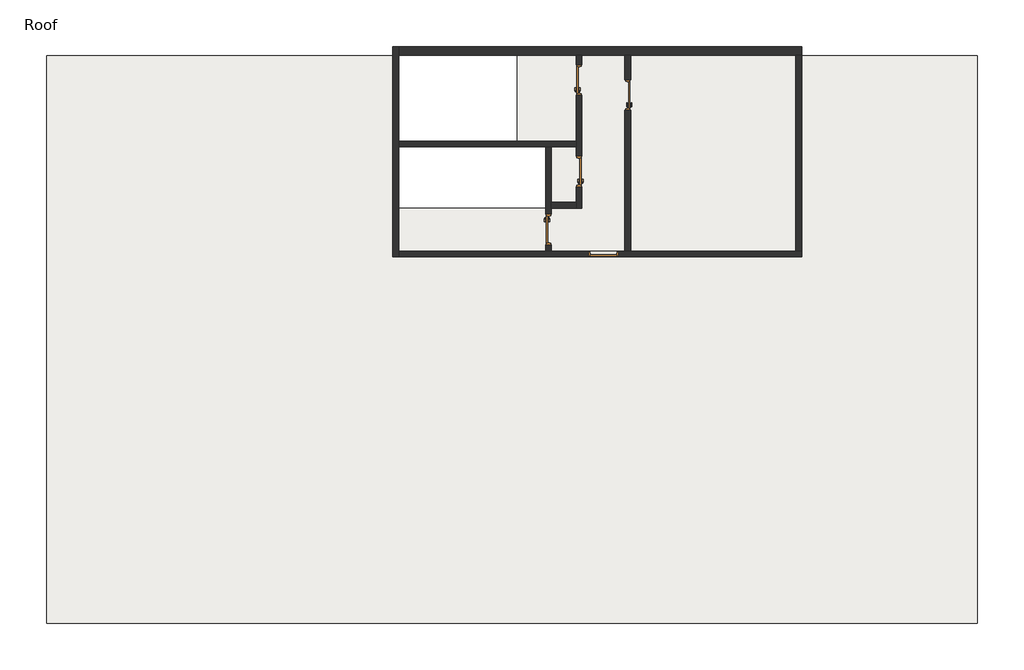
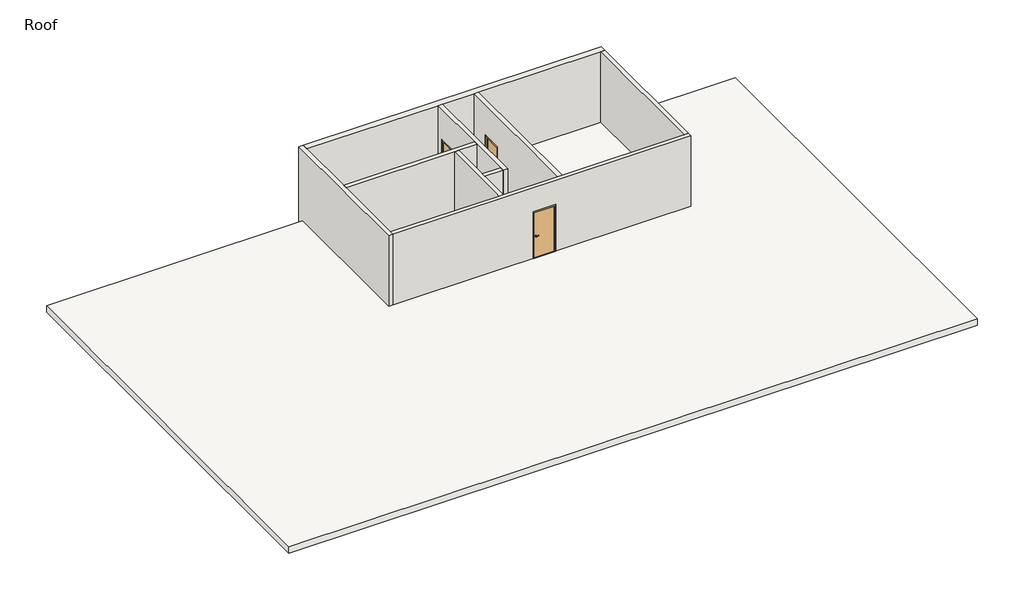
# One storey: 9 walls, 5 doors, 1 roof.
"""IFC4 building model written with IfcOpenShell, lengths in millimetres."""

import ifcopenshell
import ifcopenshell.guid

model = None  # the IFC model being written
_history = None  # IfcOwnerHistory: only IFC2X3 demands one
_inside = {}  # id of a spatial element -> (the spatial element, [elements in it])
_under = {}  # id of a project, library or spatial element -> (it, [spatial elements below it])
_declared = {}  # id of a project -> (the project, [libraries it declares])
_typed = {}  # id of a type object -> (the type object, [elements of that type])
_made_of = {}  # id of a material, layer set ... -> (it, [elements and type objects made of it])


def new_model(schema):
    """Start an empty IFC model of exactly this schema.

    Asked for "IFC4X3", IfcOpenShell would pick the latest addendum, in which some entities
    have other attributes; the version numbers below select the first issue.
    IFC2X3 requires an IfcOwnerHistory on every rooted entity: one is made here for all.
    """
    global model, _history
    if schema == "IFC4X3":
        model = ifcopenshell.file(schema_version=(4, 3, 0, 0))
    else:
        model = ifcopenshell.file(schema=schema)
    _inside.clear()
    _under.clear()
    _declared.clear()
    _typed.clear()
    _made_of.clear()
    _history = None
    if model.schema == "IFC2X3":
        org = make("IfcOrganization", Name="unknown")
        user = make(
            "IfcPersonAndOrganization",
            ThePerson=make("IfcPerson", FamilyName="unknown"),
            TheOrganization=org,
        )
        app = make(
            "IfcApplication",
            ApplicationDeveloper=org,
            Version="unknown",
            ApplicationFullName="unknown",
            ApplicationIdentifier="unknown",
        )
        _history = make(
            "IfcOwnerHistory",
            OwningUser=user,
            OwningApplication=app,
            ChangeAction="ADDED",
            CreationDate=0,
        )
    return model


def make(cls, **values):
    """One entity of the class cls with the attributes given. An attribute that is None is left unset."""
    return model.create_entity(
        cls, **{name: value for name, value in values.items() if value is not None}
    )


def rooted(cls, **values):
    """An entity with a GlobalId (a new one), such as an element, a storey or a relation."""
    return make(cls, GlobalId=ifcopenshell.guid.new(), OwnerHistory=_history, **values)


def si_unit(unit_type, name, prefix=None):
    """IfcSIUnit, for example si_unit("LENGTHUNIT", "METRE", prefix="MILLI")."""
    return make("IfcSIUnit", UnitType=unit_type, Prefix=prefix, Name=name)


def assignment(units):
    """IfcUnitAssignment: the units of a project."""
    return None if units is None else make("IfcUnitAssignment", Units=units)


def point(xyz):
    """IfcCartesianPoint."""
    return None if xyz is None else make("IfcCartesianPoint", Coordinates=xyz)


def direction(xyz):
    """IfcDirection."""
    return None if xyz is None else make("IfcDirection", DirectionRatios=xyz)


def frame(location, z_axis=None, x_axis=None):
    """IfcAxis2Placement3D, a coordinate frame: its origin and axes. An axis left out is left unset."""
    return make(
        "IfcAxis2Placement3D",
        Location=point(location),
        Axis=direction(z_axis),
        RefDirection=direction(x_axis),
    )


def frame_2d(location, x_axis=None):
    """IfcAxis2Placement2D, a coordinate frame in the plane: its origin and x axis."""
    return make(
        "IfcAxis2Placement2D", Location=point(location), RefDirection=direction(x_axis)
    )


def origin():
    """The frame at (0, 0, 0) with its axes left unset."""
    return frame((0.0, 0.0, 0.0))


def origin_with_axes():
    """The frame at (0, 0, 0) with the z axis (0, 0, 1) and the x axis (1, 0, 0) written out."""
    return frame((0.0, 0.0, 0.0), z_axis=(0.0, 0.0, 1.0), x_axis=(1.0, 0.0, 0.0))


def place(relative_to, where):
    """IfcLocalPlacement: puts the frame where relative to a parent placement (None: the world)."""
    return make(
        "IfcLocalPlacement", PlacementRelTo=relative_to, RelativePlacement=where
    )


def context(
    kind, dimensions, precision=None, world=None, true_north=None, identifier=None
):
    """IfcGeometricRepresentationContext, for example the 3D "Model" context."""
    return make(
        "IfcGeometricRepresentationContext",
        ContextIdentifier=identifier,
        ContextType=kind,
        CoordinateSpaceDimension=dimensions,
        Precision=precision,
        WorldCoordinateSystem=world,
        TrueNorth=true_north,
    )


def project(units=None, contexts=None):
    """IfcProject with its units and contexts."""
    return rooted(
        "IfcProject",
        Name="project",
        RepresentationContexts=contexts,
        UnitsInContext=assignment(units),
    )


def spatial(cls, under=None, at=None, **own):
    """A site, building, storey or space (cls), placed at a placement, below another one or the project."""
    s = rooted(cls, ObjectPlacement=at, **own)
    if under is not None:
        _under.setdefault(under.id(), (under, []))[1].append(s)
    return s


def polyline(points):
    """IfcPolyline through the points."""
    return make("IfcPolyline", Points=[point(p) for p in points])


def circle_curve(where, radius):
    """IfcCircle in the frame where."""
    return make("IfcCircle", Position=where, Radius=radius)


def ellipse_curve(where, semi_axis1, semi_axis2):
    """IfcEllipse in the frame where."""
    return make(
        "IfcEllipse", Position=where, SemiAxis1=semi_axis1, SemiAxis2=semi_axis2
    )


def trimmed(basis, trim1, trim2, sense, master):
    """IfcTrimmedCurve: the piece of a basis curve between two trims."""
    return make(
        "IfcTrimmedCurve",
        BasisCurve=basis,
        Trim1=trim1,
        Trim2=trim2,
        SenseAgreement=sense,
        MasterRepresentation=master,
    )


def segment(curve, same_sense, transition):
    """IfcCompositeCurveSegment."""
    return make(
        "IfcCompositeCurveSegment",
        Transition=transition,
        SameSense=same_sense,
        ParentCurve=curve,
    )


def composite_curve(segments, self_intersect=None):
    """IfcCompositeCurve: segments joined end to end."""
    return make("IfcCompositeCurve", Segments=segments, SelfIntersect=self_intersect)


def outline(outer, holes=None, kind="AREA"):
    """IfcArbitraryClosedProfileDef: a profile drawn as a closed curve; with holes, ...WithVoids."""
    if holes is None:
        return make("IfcArbitraryClosedProfileDef", ProfileType=kind, OuterCurve=outer)
    return make(
        "IfcArbitraryProfileDefWithVoids",
        ProfileType=kind,
        OuterCurve=outer,
        InnerCurves=holes,
    )


def extrude(swept, where, along, depth):
    """IfcExtrudedAreaSolid: the profile swept, set in the frame where, extruded along a direction by depth."""
    return make(
        "IfcExtrudedAreaSolid",
        SweptArea=swept,
        Position=where,
        ExtrudedDirection=direction(along),
        Depth=depth,
    )


def faces_of(points, faces, orient=None, outer=None):
    """IfcFace entities. A face is a list of loops; a loop is a list of indices into points, from 0.

    orient and outer hold one flag for each loop. By default every Orientation is true, the
    first loop of a face is its IfcFaceOuterBound and the others are IfcFaceBound.
    """
    made = []
    for i, loops in enumerate(faces):
        bounds = []
        for j, loop in enumerate(loops):
            is_outer = j == 0 if outer is None else outer[i][j]
            bounds.append(
                make(
                    "IfcFaceOuterBound" if is_outer else "IfcFaceBound",
                    Bound=make("IfcPolyLoop", Polygon=[points[k] for k in loop]),
                    Orientation=True if orient is None else orient[i][j],
                )
            )
        made.append(make("IfcFace", Bounds=bounds))
    return made


def faceted_brep(points, faces, orient=None, outer=None, voids=None):
    """IfcFacetedBrep: a solid bounded by flat faces; with voids (closed shells), ...WithVoids."""
    shared = [point(p) for p in points]
    hull = make("IfcClosedShell", CfsFaces=faces_of(shared, faces, orient, outer))
    if voids is None:
        return make("IfcFacetedBrep", Outer=hull)
    return make(
        "IfcFacetedBrepWithVoids",
        Outer=hull,
        Voids=[
            make(cls, CfsFaces=faces_of(shared, fs, o, b)) for cls, fs, o, b in voids
        ],
    )


def shape(context_of_items, identifier, shape_type, items):
    """IfcShapeRepresentation: the items that make up one representation, for example the "Body"."""
    return make(
        "IfcShapeRepresentation",
        ContextOfItems=context_of_items,
        RepresentationIdentifier=identifier,
        RepresentationType=shape_type,
        Items=items,
    )


def source(mapping_origin, context_of_items, identifier, shape_type, items):
    """IfcRepresentationMap: a shape defined once, which mapped items show again and again."""
    return make(
        "IfcRepresentationMap",
        MappingOrigin=mapping_origin,
        MappedRepresentation=shape(context_of_items, identifier, shape_type, items),
    )


def transform(
    local_origin,
    x_axis=None,
    y_axis=None,
    z_axis=None,
    scale=None,
    scale2=None,
    scale3=None,
    uniform=True,
):
    """IfcCartesianTransformationOperator3D, or its non-uniform kind. x_axis, y_axis, z_axis: its Axis1, 2, 3."""
    if uniform:
        return make(
            "IfcCartesianTransformationOperator3D",
            Axis1=direction(x_axis),
            Axis2=direction(y_axis),
            LocalOrigin=point(local_origin),
            Scale=scale,
            Axis3=direction(z_axis),
        )
    return make(
        "IfcCartesianTransformationOperator3DnonUniform",
        Axis1=direction(x_axis),
        Axis2=direction(y_axis),
        LocalOrigin=point(local_origin),
        Scale=scale,
        Axis3=direction(z_axis),
        Scale2=scale2,
        Scale3=scale3,
    )


def mapped(mapping_source, mapping_target):
    """IfcMappedItem: shows the shape of a source again, moved by a transform."""
    return make(
        "IfcMappedItem", MappingSource=mapping_source, MappingTarget=mapping_target
    )


def made_of(thing, what):
    """Note that an element or type object is made of a material, layer set ...; save() writes the relation."""
    if what is not None:
        _made_of.setdefault(what.id(), (what, []))[1].append(thing)
    return thing


def element(
    cls,
    number,
    at=None,
    inside=None,
    cuts=None,
    type_object=None,
    material=None,
    context=None,
    identifier="Body",
    shape_type=None,
    held_by="IfcProductDefinitionShape",
    body=None,
    shapes=None,
    **own,
):
    """One element of the class cls, such as IfcWall. Its Tag is "e" and its number.

    at: its placement. inside: the storey or other place that contains it. cuts: it is an
    opening in that element (IfcRelVoidsElement). A single representation is given by context,
    identifier, shape_type and body (its items); several are given by shapes. held_by: the class
    of the entity that holds the representations. save() writes the other relations.
    """
    e = rooted(cls, Tag="e%d" % number, ObjectPlacement=at, **own)
    if body is not None:
        shapes = [shape(context, identifier, shape_type, body)]
    if shapes is not None:
        e.Representation = make(held_by, Representations=shapes)
    if inside is not None:
        _inside.setdefault(inside.id(), (inside, []))[1].append(e)
    if cuts is not None:
        rooted(
            "IfcRelVoidsElement", RelatingBuildingElement=cuts, RelatedOpeningElement=e
        )
    if type_object is not None:
        _typed.setdefault(type_object.id(), (type_object, []))[1].append(e)
    return made_of(e, material)


def aggregate(whole, parts):
    """IfcRelAggregates: a whole, such as a stair, and the parts it consists of."""
    return rooted("IfcRelAggregates", RelatingObject=whole, RelatedObjects=parts)


def save(model, path):
    """Write the relations noted so far, then the file.

    IfcRelAggregates (storeys below a building ...), IfcRelContainedInSpatialStructure (elements
    in a storey), IfcRelDefinesByType, IfcRelAssociatesMaterial and IfcRelDeclares: one each for
    every whole, place, type object, material and project.
    """
    for whole, parts in _under.values():
        aggregate(whole, parts)
    for where, things in _inside.values():
        rooted(
            "IfcRelContainedInSpatialStructure",
            RelatedElements=things,
            RelatingStructure=where,
        )
    for kind, things in _typed.values():
        rooted("IfcRelDefinesByType", RelatedObjects=things, RelatingType=kind)
    for what, things in _made_of.values():
        rooted("IfcRelAssociatesMaterial", RelatedObjects=things, RelatingMaterial=what)
    for by, libraries in _declared.values():
        rooted("IfcRelDeclares", RelatingContext=by, RelatedDefinitions=libraries)
    model.write(path)


def plane_surface(at):
    """IfcPlane: the flat surface through the origin of the frame at, square to its z axis."""
    return make("IfcPlane", Position=at)


def cylinder_surface(at, radius):
    """IfcCylindricalSurface: all points at the distance radius from the z axis of the frame at."""
    return make("IfcCylindricalSurface", Position=at, Radius=radius)


def revolved_surface(curve, axis_point, axis_direction):
    """IfcSurfaceOfRevolution: the curve turned about the line through axis_point along axis_direction."""
    return make(
        "IfcSurfaceOfRevolution",
        SweptCurve=make("IfcArbitraryOpenProfileDef", ProfileType="CURVE", Curve=curve),
        AxisPosition=make("IfcAxis1Placement", Location=point(axis_point), Axis=direction(axis_direction)),
    )


def advanced_brep(points, edges, surfaces, faces):
    """IfcAdvancedBrep: a solid bounded by faces that lie on surfaces and meet in shared edges.

    An edge is (start, end): straight between two places in points (the first is 0);
    or (start, end, curve); or (start, end, curve, False) where it runs against its curve.
    A face is (place in surfaces, loops), or (place, loops, False) where it looks against
    its surface's normal. A loop lists edges by number (the first is 1), with a minus sign
    where the edge is run from its end to its start. The first loop is the outer one.
    """
    corners = [point(p) for p in points]
    vertices = [make("IfcVertexPoint", VertexGeometry=c) for c in corners]
    made = []
    for start, end, *more in edges:
        made.append(
            make(
                "IfcEdgeCurve",
                EdgeStart=vertices[start],
                EdgeEnd=vertices[end],
                EdgeGeometry=more[0] if more else make("IfcPolyline", Points=[corners[start], corners[end]]),
                SameSense=more[1] if len(more) > 1 else True,
            )
        )
    hull = []
    for where, loops, *sense in faces:
        bounds = []
        for j, loop in enumerate(loops):
            ring = [make("IfcOrientedEdge", EdgeElement=made[abs(k) - 1], Orientation=k > 0) for k in loop]
            bounds.append(
                make(
                    "IfcFaceOuterBound" if j == 0 else "IfcFaceBound",
                    Bound=make("IfcEdgeLoop", EdgeList=ring),
                    Orientation=True,
                )
            )
        hull.append(make("IfcAdvancedFace", Bounds=bounds, FaceSurface=surfaces[where], SameSense=sense[0] if sense else True))
    return make("IfcAdvancedBrep", Outer=make("IfcClosedShell", CfsFaces=hull))


def door_9f6fe377(model_context):
    return source(origin(), model_context, "Body", "SolidModel", [
        advanced_brep(
        [(-392.190625, -25.3375, 1016.0), (-372.190625, -25.3375, 1016.0), (-392.190625, 4.6625, 1016.0), (-372.190625, 4.6625, 1016.0), (-367.190625, 9.6625, 1016.0), (-367.190625, 29.6625, 1016.0), (-262.190625, 29.6625, 1016.0), (-262.190625, 9.6625, 1016.0)],
        [
            (0, 1, circle_curve(frame((-382.190625, -25.3375, 1016.0), z_axis=(0.0, -1.0, 0.0), x_axis=(1.0, 0.0, 0.0)), 10.0)),
            (1, 0, circle_curve(frame((-382.190625, -25.3375, 1016.0), z_axis=(0.0, -1.0, 0.0), x_axis=(1.0, 0.0, 0.0)), 10.0)),
            (0, 2),
            (2, 3, circle_curve(frame((-382.190625, 4.6625, 1016.0), z_axis=(0.0, -1.0, 0.0), x_axis=(1.0, 0.0, 0.0)), 10.0)),
            (3, 1),
            (3, 2, circle_curve(frame((-382.190625, 4.6625, 1016.0), z_axis=(0.0, -1.0, 0.0), x_axis=(1.0, 0.0, 0.0)), 10.0)),
            (4, 3, circle_curve(frame((-367.190625, 4.6625, 1016.0), z_axis=(0.0, 0.0, 1.0), x_axis=(-1.0, 0.0, 0.0)), 5.0)),
            (2, 5, circle_curve(frame((-367.190625, 4.6625, 1016.0), z_axis=(0.0, 0.0, -1.0), x_axis=(-1.0, 0.0, 0.0)), 25.0)),
            (5, 4, circle_curve(frame((-367.190625, 19.6625, 1016.0), z_axis=(-1.0, 0.0, 0.0), x_axis=(0.0, -1.0, 0.0)), 10.0)),
            (4, 5, circle_curve(frame((-367.190625, 19.6625, 1016.0), z_axis=(-1.0, 0.0, 0.0), x_axis=(0.0, -1.0, 0.0)), 10.0)),
            (6, 7, circle_curve(frame((-262.190625, 19.6625, 1016.0), z_axis=(1.0, 0.0, 0.0), x_axis=(0.0, -1.0, 0.0)), 10.0)),
            (7, 6, circle_curve(frame((-262.190625, 19.6625, 1016.0), z_axis=(1.0, 0.0, 0.0), x_axis=(0.0, -1.0, 0.0)), 10.0)),
            (5, 6),
            (7, 4),
        ],
        [
            plane_surface(frame((-382.190625, -25.3375, 1016.0), z_axis=(0.0, -1.0, 0.0), x_axis=(0.0, 0.0, 1.0))),
            cylinder_surface(frame((-382.190625, -25.3375, 1016.0), z_axis=(0.0, -1.0, 0.0), x_axis=(1.0, 0.0, 0.0)), 10.0),
            revolved_surface(trimmed(ellipse_curve(frame((-382.190625, 4.6625, 1016.0), z_axis=(0.0, -1.0, 0.0), x_axis=(1.0, 0.0, 0.0)), 10.0, 10.0), [point((-392.190625, 4.6625, 1016.0))], [point((-372.190625, 4.6625, 1016.0))], True, "CARTESIAN"), (-367.190625, 4.6625, 1016.0), (0.0, 0.0, -1.0)),
            revolved_surface(trimmed(ellipse_curve(frame((-382.190625, 4.6625, 1016.0), z_axis=(0.0, -1.0, 0.0), x_axis=(1.0, 0.0, 0.0)), 10.0, 10.0), [point((-372.190625, 4.6625, 1016.0))], [point((-392.190625, 4.6625, 1016.0))], True, "CARTESIAN"), (-367.190625, 4.6625, 1016.0), (0.0, 0.0, -1.0)),
            plane_surface(frame((-262.190625, 19.6625, 1016.0), z_axis=(1.0, 0.0, 0.0), x_axis=(0.0, 0.0, 1.0))),
            cylinder_surface(frame((-367.190625, 19.6625, 1016.0), z_axis=(-1.0, 0.0, 0.0), x_axis=(0.0, -1.0, 0.0)), 10.0),
        ],
        [
            (0, [[1, 2]]),
            (1, [[-1, 3, 4, 5]]),
            (1, [[-2, -5, 6, -3]]),
            (2, [[7, -4, 8, 9]]),
            (3, [[-8, -6, -7, 10]]),
            (4, [[11, 12]]),
            (5, [[-9, 13, -12, 14]]),
            (5, [[-10, -14, -11, -13]]),
        ],
    ),
        extrude(outline(composite_curve([segment(trimmed(circle_curve(frame_2d((1016.0, -384.690625)), 30.0), [point((1016.0, -414.690625))], [point((1016.0, -354.690625))], False, "CARTESIAN"), True, "CONTINUOUS"), segment(trimmed(circle_curve(frame_2d((1016.0, -384.690625)), 30.0), [point((1016.0, -354.690625))], [point((1016.0, -414.690625))], False, "CARTESIAN"), True, "CONTINUOUS")], self_intersect=False)), frame((0.0, -33.3375, 0.0), z_axis=(0.0, 1.0, 0.0), x_axis=(0.0, 0.0, 1.0)), (0.0, 0.0, 1.0), 8.0),
        advanced_brep(
        [(-392.190625, -85.7875, 1016.0), (-372.190625, -85.7875, 1016.0), (-372.190625, -115.7875, 1016.0), (-392.190625, -115.7875, 1016.0), (-367.190625, -120.7875, 1016.0), (-367.190625, -140.7875, 1016.0), (-262.190625, -140.7875, 1016.0), (-262.190625, -120.7875, 1016.0)],
        [
            (0, 1, circle_curve(frame((-382.190625, -85.7875, 1016.0), z_axis=(0.0, 1.0, 0.0), x_axis=(1.0, 0.0, 0.0)), 10.0)),
            (1, 0, circle_curve(frame((-382.190625, -85.7875, 1016.0), z_axis=(0.0, 1.0, 0.0), x_axis=(1.0, 0.0, 0.0)), 10.0)),
            (1, 2),
            (2, 3, circle_curve(frame((-382.190625, -115.7875, 1016.0), z_axis=(0.0, 1.0, 0.0), x_axis=(1.0, 0.0, 0.0)), 10.0)),
            (3, 0),
            (3, 2, circle_curve(frame((-382.190625, -115.7875, 1016.0), z_axis=(0.0, 1.0, 0.0), x_axis=(1.0, 0.0, 0.0)), 10.0)),
            (4, 5, circle_curve(frame((-367.190625, -130.7875, 1016.0), z_axis=(-1.0, 0.0, 0.0), x_axis=(0.0, 1.0, 0.0)), 10.0)),
            (5, 3, circle_curve(frame((-367.190625, -115.7875, 1016.0), z_axis=(0.0, 0.0, -1.0), x_axis=(-1.0, 0.0, 0.0)), 25.0)),
            (2, 4, circle_curve(frame((-367.190625, -115.7875, 1016.0), z_axis=(0.0, 0.0, 1.0), x_axis=(-1.0, 0.0, 0.0)), 5.0)),
            (5, 4, circle_curve(frame((-367.190625, -130.7875, 1016.0), z_axis=(-1.0, 0.0, 0.0), x_axis=(0.0, 1.0, 0.0)), 10.0)),
            (6, 7, circle_curve(frame((-262.190625, -130.7875, 1016.0), z_axis=(1.0, 0.0, 0.0), x_axis=(0.0, 1.0, 0.0)), 10.0)),
            (7, 6, circle_curve(frame((-262.190625, -130.7875, 1016.0), z_axis=(1.0, 0.0, 0.0), x_axis=(0.0, 1.0, 0.0)), 10.0)),
            (4, 7),
            (6, 5),
        ],
        [
            plane_surface(frame((-382.190625, -85.7875, 1016.0), z_axis=(0.0, 1.0, 0.0), x_axis=(0.0, 0.0, 1.0))),
            cylinder_surface(frame((-382.190625, -85.7875, 1016.0), z_axis=(0.0, 1.0, 0.0), x_axis=(1.0, 0.0, 0.0)), 10.0),
            revolved_surface(trimmed(ellipse_curve(frame((-382.190625, -115.7875, 1016.0), z_axis=(0.0, -1.0, 0.0), x_axis=(1.0, 0.0, 0.0)), 10.0, 10.0), [point((-392.190625, -115.7875, 1016.0))], [point((-372.190625, -115.7875, 1016.0))], True, "CARTESIAN"), (-367.190625, -115.7875, 1016.0), (0.0, 0.0, -1.0)),
            revolved_surface(trimmed(ellipse_curve(frame((-382.190625, -115.7875, 1016.0), z_axis=(0.0, -1.0, 0.0), x_axis=(1.0, 0.0, 0.0)), 10.0, 10.0), [point((-372.190625, -115.7875, 1016.0))], [point((-392.190625, -115.7875, 1016.0))], True, "CARTESIAN"), (-367.190625, -115.7875, 1016.0), (0.0, 0.0, -1.0)),
            plane_surface(frame((-262.190625, -130.7875, 1016.0), z_axis=(1.0, 0.0, 0.0), x_axis=(0.0, 0.0, 1.0))),
            cylinder_surface(frame((-367.190625, -130.7875, 1016.0), z_axis=(-1.0, 0.0, 0.0), x_axis=(0.0, 1.0, 0.0)), 10.0),
        ],
        [
            (0, [[1, 2]]),
            (1, [[3, 4, 5, -2]]),
            (1, [[-5, 6, -3, -1]]),
            (2, [[7, 8, -4, 9]]),
            (3, [[10, -9, -6, -8]]),
            (4, [[11, 12]]),
            (5, [[13, -11, 14, -7]]),
            (5, [[-14, -12, -13, -10]]),
        ],
    ),
        extrude(outline(composite_curve([segment(trimmed(circle_curve(frame_2d((1016.0, -384.690625)), 30.0), [point((1016.0, -414.690625))], [point((1016.0, -354.690625))], False, "CARTESIAN"), True, "CONTINUOUS"), segment(trimmed(circle_curve(frame_2d((1016.0, -384.690625)), 30.0), [point((1016.0, -354.690625))], [point((1016.0, -414.690625))], False, "CARTESIAN"), True, "CONTINUOUS")], self_intersect=False)), frame((0.0, -85.7875, 0.0), z_axis=(0.0, 1.0, 0.0), x_axis=(0.0, 0.0, 1.0)), (0.0, 0.0, 1.0), 8.0),
        faceted_brep([(457.2, -28.575, 0.0), (441.325, -28.575, 0.0), (441.325, 19.05, 0.0), (457.2, 19.05, 0.0), (457.2, 68.2625, 0.0), (508.0, 68.2625, 0.0), (508.0, -77.7875, 0.0), (457.2, -77.7875, 0.0), (457.2, -77.7875, 2133.6), (457.2, -28.575, 2133.6), (508.0, -77.7875, 2235.2), (-508.0, -77.7875, 2235.2), (-508.0, -77.7875, 0.0), (-457.2, -77.7875, 0.0), (-457.2, -77.7875, 2133.6), (508.0, 68.2625, 2235.2), (457.2, 68.2625, 2133.6), (-457.2, 68.2625, 2133.6), (-457.2, 68.2625, 0.0), (-508.0, 68.2625, 0.0), (-508.0, 68.2625, 2235.2), (457.2, 19.05, 2133.6), (441.325, 19.05, 2117.725), (-441.325, 19.05, 2117.725), (-441.325, 19.05, 0.0), (-457.2, 19.05, 0.0), (-457.2, 19.05, 2133.6), (441.325, -28.575, 2117.725), (-457.2, -28.575, 2133.6), (-457.2, -28.575, 0.0), (-441.325, -28.575, 0.0), (-441.325, -28.575, 2117.725)], [[[0, 1, 2, 3, 4, 5, 6, 7]], [[7, 8, 9, 0]], [[6, 10, 11, 12, 13, 14, 8, 7]], [[5, 15, 10, 6]], [[4, 16, 17, 18, 19, 20, 15, 5]], [[3, 21, 16, 4]], [[2, 22, 23, 24, 25, 26, 21, 3]], [[1, 27, 22, 2]], [[0, 9, 28, 29, 30, 31, 27, 1]], [[8, 14, 28, 9]], [[16, 21, 26, 17]], [[22, 27, 31, 23]], [[12, 19, 18, 25, 24, 30, 29, 13]], [[13, 29, 28, 14]], [[11, 20, 19, 12]], [[17, 26, 25, 18]], [[23, 31, 30, 24]], [[15, 20, 11, 10]]]),
        extrude(outline(polyline([(457.2, -33.3375), (457.2, -77.7875), (-457.2, -77.7875), (-457.2, -33.3375), (457.2, -33.3375)])), origin_with_axes(), (0.0, 0.0, 1.0), 2133.6),
    ])


def door_87fe937e(model_context):
    return source(origin(), model_context, "Body", "SolidModel", [
        advanced_brep(
        [(-392.190625, 25.3375, 1016.0), (-372.190625, 25.3375, 1016.0), (-372.190625, -4.6625, 1016.0), (-392.190625, -4.6625, 1016.0), (-367.190625, -9.6625, 1016.0), (-367.190625, -29.6625, 1016.0), (-262.190625, -29.6625, 1016.0), (-262.190625, -9.6625, 1016.0)],
        [
            (0, 1, circle_curve(frame((-382.190625, 25.3375, 1016.0), z_axis=(0.0, 1.0, 0.0), x_axis=(1.0, 0.0, 0.0)), 10.0)),
            (1, 0, circle_curve(frame((-382.190625, 25.3375, 1016.0), z_axis=(0.0, 1.0, 0.0), x_axis=(1.0, 0.0, 0.0)), 10.0)),
            (1, 2),
            (2, 3, circle_curve(frame((-382.190625, -4.6625, 1016.0), z_axis=(0.0, 1.0, 0.0), x_axis=(1.0, 0.0, 0.0)), 10.0)),
            (3, 0),
            (3, 2, circle_curve(frame((-382.190625, -4.6625, 1016.0), z_axis=(0.0, 1.0, 0.0), x_axis=(1.0, 0.0, 0.0)), 10.0)),
            (4, 5, circle_curve(frame((-367.190625, -19.6625, 1016.0), z_axis=(-1.0, 0.0, 0.0), x_axis=(0.0, 1.0, 0.0)), 10.0)),
            (5, 3, circle_curve(frame((-367.190625, -4.6625, 1016.0), z_axis=(0.0, 0.0, -1.0), x_axis=(-1.0, 0.0, 0.0)), 25.0)),
            (2, 4, circle_curve(frame((-367.190625, -4.6625, 1016.0), z_axis=(0.0, 0.0, 1.0), x_axis=(-1.0, 0.0, 0.0)), 5.0)),
            (5, 4, circle_curve(frame((-367.190625, -19.6625, 1016.0), z_axis=(-1.0, 0.0, 0.0), x_axis=(0.0, 1.0, 0.0)), 10.0)),
            (6, 7, circle_curve(frame((-262.190625, -19.6625, 1016.0), z_axis=(1.0, 0.0, 0.0), x_axis=(0.0, 1.0, 0.0)), 10.0)),
            (7, 6, circle_curve(frame((-262.190625, -19.6625, 1016.0), z_axis=(1.0, 0.0, 0.0), x_axis=(0.0, 1.0, 0.0)), 10.0)),
            (4, 7),
            (6, 5),
        ],
        [
            plane_surface(frame((-382.190625, 25.3375, 1016.0), z_axis=(0.0, 1.0, 0.0), x_axis=(0.0, 0.0, 1.0))),
            cylinder_surface(frame((-382.190625, 25.3375, 1016.0), z_axis=(0.0, 1.0, 0.0), x_axis=(1.0, 0.0, 0.0)), 10.0),
            revolved_surface(trimmed(ellipse_curve(frame((-382.190625, -4.6625, 1016.0), z_axis=(0.0, -1.0, 0.0), x_axis=(1.0, 0.0, 0.0)), 10.0, 10.0), [point((-392.190625, -4.6625, 1016.0))], [point((-372.190625, -4.6625, 1016.0))], True, "CARTESIAN"), (-367.190625, -4.6625, 1016.0), (0.0, 0.0, -1.0)),
            revolved_surface(trimmed(ellipse_curve(frame((-382.190625, -4.6625, 1016.0), z_axis=(0.0, -1.0, 0.0), x_axis=(1.0, 0.0, 0.0)), 10.0, 10.0), [point((-372.190625, -4.6625, 1016.0))], [point((-392.190625, -4.6625, 1016.0))], True, "CARTESIAN"), (-367.190625, -4.6625, 1016.0), (0.0, 0.0, -1.0)),
            plane_surface(frame((-262.190625, -19.6625, 1016.0), z_axis=(1.0, 0.0, 0.0), x_axis=(0.0, 0.0, 1.0))),
            cylinder_surface(frame((-367.190625, -19.6625, 1016.0), z_axis=(-1.0, 0.0, 0.0), x_axis=(0.0, 1.0, 0.0)), 10.0),
        ],
        [
            (0, [[1, 2]]),
            (1, [[3, 4, 5, -2]]),
            (1, [[-5, 6, -3, -1]]),
            (2, [[7, 8, -4, 9]]),
            (3, [[10, -9, -6, -8]]),
            (4, [[11, 12]]),
            (5, [[13, -11, 14, -7]]),
            (5, [[-14, -12, -13, -10]]),
        ],
    ),
        extrude(outline(composite_curve([segment(trimmed(circle_curve(frame_2d((1016.0, -384.690625)), 30.0), [point((1016.0, -414.690625))], [point((1016.0, -354.690625))], False, "CARTESIAN"), True, "CONTINUOUS"), segment(trimmed(circle_curve(frame_2d((1016.0, -384.690625)), 30.0), [point((1016.0, -354.690625))], [point((1016.0, -414.690625))], False, "CARTESIAN"), True, "CONTINUOUS")], self_intersect=False)), frame((0.0, 25.3375, 0.0), z_axis=(0.0, 1.0, 0.0), x_axis=(0.0, 0.0, 1.0)), (0.0, 0.0, 1.0), 8.0),
        advanced_brep(
        [(-392.190625, 85.7875, 1016.0), (-372.190625, 85.7875, 1016.0), (-392.190625, 115.7875, 1016.0), (-372.190625, 115.7875, 1016.0), (-367.190625, 120.7875, 1016.0), (-367.190625, 140.7875, 1016.0), (-262.190625, 140.7875, 1016.0), (-262.190625, 120.7875, 1016.0)],
        [
            (0, 1, circle_curve(frame((-382.190625, 85.7875, 1016.0), z_axis=(0.0, -1.0, 0.0), x_axis=(1.0, 0.0, 0.0)), 10.0)),
            (1, 0, circle_curve(frame((-382.190625, 85.7875, 1016.0), z_axis=(0.0, -1.0, 0.0), x_axis=(1.0, 0.0, 0.0)), 10.0)),
            (0, 2),
            (2, 3, circle_curve(frame((-382.190625, 115.7875, 1016.0), z_axis=(0.0, -1.0, 0.0), x_axis=(1.0, 0.0, 0.0)), 10.0)),
            (3, 1),
            (3, 2, circle_curve(frame((-382.190625, 115.7875, 1016.0), z_axis=(0.0, -1.0, 0.0), x_axis=(1.0, 0.0, 0.0)), 10.0)),
            (4, 3, circle_curve(frame((-367.190625, 115.7875, 1016.0), z_axis=(0.0, 0.0, 1.0), x_axis=(-1.0, 0.0, 0.0)), 5.0)),
            (2, 5, circle_curve(frame((-367.190625, 115.7875, 1016.0), z_axis=(0.0, 0.0, -1.0), x_axis=(-1.0, 0.0, 0.0)), 25.0)),
            (5, 4, circle_curve(frame((-367.190625, 130.7875, 1016.0), z_axis=(-1.0, 0.0, 0.0), x_axis=(0.0, -1.0, 0.0)), 10.0)),
            (4, 5, circle_curve(frame((-367.190625, 130.7875, 1016.0), z_axis=(-1.0, 0.0, 0.0), x_axis=(0.0, -1.0, 0.0)), 10.0)),
            (6, 7, circle_curve(frame((-262.190625, 130.7875, 1016.0), z_axis=(1.0, 0.0, 0.0), x_axis=(0.0, -1.0, 0.0)), 10.0)),
            (7, 6, circle_curve(frame((-262.190625, 130.7875, 1016.0), z_axis=(1.0, 0.0, 0.0), x_axis=(0.0, -1.0, 0.0)), 10.0)),
            (5, 6),
            (7, 4),
        ],
        [
            plane_surface(frame((-382.190625, 85.7875, 1016.0), z_axis=(0.0, -1.0, 0.0), x_axis=(0.0, 0.0, 1.0))),
            cylinder_surface(frame((-382.190625, 85.7875, 1016.0), z_axis=(0.0, -1.0, 0.0), x_axis=(1.0, 0.0, 0.0)), 10.0),
            revolved_surface(trimmed(ellipse_curve(frame((-382.190625, 115.7875, 1016.0), z_axis=(0.0, -1.0, 0.0), x_axis=(1.0, 0.0, 0.0)), 10.0, 10.0), [point((-392.190625, 115.7875, 1016.0))], [point((-372.190625, 115.7875, 1016.0))], True, "CARTESIAN"), (-367.190625, 115.7875, 1016.0), (0.0, 0.0, -1.0)),
            revolved_surface(trimmed(ellipse_curve(frame((-382.190625, 115.7875, 1016.0), z_axis=(0.0, -1.0, 0.0), x_axis=(1.0, 0.0, 0.0)), 10.0, 10.0), [point((-372.190625, 115.7875, 1016.0))], [point((-392.190625, 115.7875, 1016.0))], True, "CARTESIAN"), (-367.190625, 115.7875, 1016.0), (0.0, 0.0, -1.0)),
            plane_surface(frame((-262.190625, 130.7875, 1016.0), z_axis=(1.0, 0.0, 0.0), x_axis=(0.0, 0.0, 1.0))),
            cylinder_surface(frame((-367.190625, 130.7875, 1016.0), z_axis=(-1.0, 0.0, 0.0), x_axis=(0.0, -1.0, 0.0)), 10.0),
        ],
        [
            (0, [[1, 2]]),
            (1, [[-1, 3, 4, 5]]),
            (1, [[-2, -5, 6, -3]]),
            (2, [[7, -4, 8, 9]]),
            (3, [[-8, -6, -7, 10]]),
            (4, [[11, 12]]),
            (5, [[-9, 13, -12, 14]]),
            (5, [[-10, -14, -11, -13]]),
        ],
    ),
        extrude(outline(composite_curve([segment(trimmed(circle_curve(frame_2d((1016.0, -384.690625)), 30.0), [point((1016.0, -414.690625))], [point((1016.0, -354.690625))], False, "CARTESIAN"), True, "CONTINUOUS"), segment(trimmed(circle_curve(frame_2d((1016.0, -384.690625)), 30.0), [point((1016.0, -354.690625))], [point((1016.0, -414.690625))], False, "CARTESIAN"), True, "CONTINUOUS")], self_intersect=False)), frame((0.0, 77.7875, 0.0), z_axis=(0.0, 1.0, 0.0), x_axis=(0.0, 0.0, 1.0)), (0.0, 0.0, 1.0), 8.0),
        faceted_brep([(457.2, 28.575, 0.0), (457.2, 77.7875, 0.0), (508.0, 77.7875, 0.0), (508.0, -68.2625, 0.0), (457.2, -68.2625, 0.0), (457.2, -19.05, 0.0), (441.325, -19.05, 0.0), (441.325, 28.575, 0.0), (457.2, 28.575, 2133.6), (457.2, 77.7875, 2133.6), (-457.2, 77.7875, 2133.6), (-457.2, 77.7875, 0.0), (-508.0, 77.7875, 0.0), (-508.0, 77.7875, 2235.2), (508.0, 77.7875, 2235.2), (508.0, -68.2625, 2235.2), (-508.0, -68.2625, 2235.2), (-508.0, -68.2625, 0.0), (-457.2, -68.2625, 0.0), (-457.2, -68.2625, 2133.6), (457.2, -68.2625, 2133.6), (457.2, -19.05, 2133.6), (-457.2, -19.05, 2133.6), (-457.2, -19.05, 0.0), (-441.325, -19.05, 0.0), (-441.325, -19.05, 2117.725), (441.325, -19.05, 2117.725), (441.325, 28.575, 2117.725), (-441.325, 28.575, 2117.725), (-441.325, 28.575, 0.0), (-457.2, 28.575, 0.0), (-457.2, 28.575, 2133.6)], [[[0, 1, 2, 3, 4, 5, 6, 7]], [[1, 0, 8, 9]], [[2, 1, 9, 10, 11, 12, 13, 14]], [[3, 2, 14, 15]], [[4, 3, 15, 16, 17, 18, 19, 20]], [[5, 4, 20, 21]], [[6, 5, 21, 22, 23, 24, 25, 26]], [[7, 6, 26, 27]], [[0, 7, 27, 28, 29, 30, 31, 8]], [[9, 8, 31, 10]], [[20, 19, 22, 21]], [[26, 25, 28, 27]], [[12, 11, 30, 29, 24, 23, 18, 17]], [[11, 10, 31, 30]], [[13, 12, 17, 16]], [[19, 18, 23, 22]], [[25, 24, 29, 28]], [[15, 14, 13, 16]]]),
        extrude(outline(polyline([(457.2, 33.3375), (-457.2, 33.3375), (-457.2, 77.7875), (457.2, 77.7875), (457.2, 33.3375)])), origin_with_axes(), (0.0, 0.0, 1.0), 2133.6),
    ])


model = new_model("IFC4")

# Units and contexts
model_context = context("Model", 3, world=origin())
ifc_project = project(units=[si_unit("LENGTHUNIT", "METRE", prefix="MILLI")], contexts=[model_context])

# Site, building, storey
site = spatial("IfcSite", under=ifc_project)
building = spatial("IfcBuilding", under=site)
storey = spatial("IfcBuildingStorey", under=building, Name="Roof", Elevation=14630.4)

# Doors
placement = place(None, origin())
door_shape = door_9f6fe377(model_context)
element("IfcDoor", 1, ObjectType="Door-Passage-Single-Flush : 36\" x 84\"", at=placement, inside=storey, context=model_context, shape_type="MappedRepresentation", body=[
    mapped(door_shape, transform((1058.2752268, 5440.2265304, 14630.4), x_axis=(0.0, 1.0, 0.0), y_axis=(-1.0, 0.0, 0.0), z_axis=(0.0, 0.0, 1.0))),
])
element("IfcDoor", 2, ObjectType="Door-Passage-Single-Flush : 36\" x 84\"", at=placement, inside=storey, context=model_context, shape_type="MappedRepresentation", body=[
    mapped(door_shape, transform((54.9752268, 3500.3015304, 14630.4), x_axis=(0.0, -1.0, 0.0), y_axis=(1.0, 0.0, 0.0), z_axis=(0.0, 0.0, 1.0))),
])
element("IfcDoor", 3, ObjectType="Door-Passage-Single-Flush : 36\" x 84\"", at=placement, inside=storey, context=model_context, shape_type="MappedRepresentation", body=[
    mapped(door_shape, transform((2683.8752268, 7980.2265304, 14630.4), x_axis=(0.0, 1.0, 0.0), y_axis=(-1.0, 0.0, 0.0), z_axis=(0.0, 0.0, 1.0))),
])
element("IfcDoor", 4, ObjectType="Door-Passage-Single-Flush : 36\" x 84\"", at=placement, inside=storey, context=model_context, shape_type="MappedRepresentation", body=[
    mapped(door_shape, transform((1877.4252268, 2698.6140304, 14935.2), x_axis=(1.0, 0.0, 0.0), y_axis=(0.0, 1.0, 0.0), z_axis=(0.0, 0.0, 1.0))),
])
door_2_shape = door_87fe937e(model_context)
element("IfcDoor", 5, ObjectType="Door-Passage-Single-Flush : 36\" x 84\"", at=placement, inside=storey, context=model_context, shape_type="MappedRepresentation", body=[
    mapped(door_2_shape, transform((1070.9752268, 8488.2265304, 14630.4), x_axis=(0.0, 1.0, 0.0), y_axis=(-1.0, 0.0, 0.0), z_axis=(0.0, 0.0, 1.0))),
])

# Roof
element("IfcRoof", 6, ObjectType="Generic - 12\"", at=placement, inside=storey, context=model_context, shape_type="SweptSolid", body=[
    extrude(outline(polyline([(14328.1877268, 9291.5015304), (14328.1877268, -9606.0984696), (-16659.8122732, -9606.0984696), (-16659.8122732, 9291.5015304), (-5128.2122732, 9291.5015304), (-5128.2122732, 4221.0265304), (145.4627268, 4221.0265304), (145.4627268, 6446.7015304), (-988.0122732, 6446.7015304), (-988.0122732, 9291.5015304), (14328.1877268, 9291.5015304)])), frame((0.0, 0.0, 14630.4), z_axis=(0.0, 0.0, 1.0), x_axis=(1.0, 0.0, 0.0)), (0.0, 0.0, 1.0), 304.8),
])

# Walls
element("IfcWall", 7, ObjectType="Generic - 12\" Masonry", at=placement, inside=storey, context=model_context, shape_type="Brep", body=[
    faceted_brep([(-4934.5372732, 9301.0265304, 18288.0), (-4934.5372732, 9301.0265304, 14630.4), (967.7877268, 9301.0265304, 14630.4), (1161.4627268, 9301.0265304, 14630.4), (2593.3877268, 9301.0265304, 14630.4), (2787.0627268, 9301.0265304, 14630.4), (8282.9877268, 9301.0265304, 14630.4), (8476.6627268, 9301.0265304, 14630.4), (8476.6627268, 9301.0265304, 18288.0), (8282.9877268, 9301.0265304, 18288.0), (2787.0627268, 9301.0265304, 18288.0), (2593.3877268, 9301.0265304, 18288.0), (1161.4627268, 9301.0265304, 18288.0), (967.7877268, 9301.0265304, 18288.0), (-4934.5372732, 9596.3015304, 14630.4), (-4934.5372732, 9596.3015304, 18288.0), (8476.6627268, 9596.3015304, 18288.0), (8476.6627268, 9596.3015304, 14630.4), (8282.9877268, 9596.3015304, 14630.4)], [[[0, 1, 2, 3, 4, 5, 6, 7, 8, 9, 10, 11, 12, 13]], [[14, 15, 16, 17, 18]], [[7, 6, 5, 4, 3, 2, 1, 14, 18, 17]], [[0, 13, 12, 11, 10, 9, 8, 16, 15]], [[0, 15, 14, 1]], [[7, 17, 16, 8]]]),
])
element("IfcWall", 8, ObjectType="Generic - 8\" Masonry", at=placement, inside=storey, context=model_context, shape_type="Brep", body=[
    faceted_brep([(-5128.2122732, 9596.3015304, 18288.0), (-5128.2122732, 9596.3015304, 14630.4), (-5128.2122732, 2595.4265304, 14630.4), (-5128.2122732, 2595.4265304, 18288.0), (-4934.5372732, 9596.3015304, 14630.4), (-4934.5372732, 9596.3015304, 18288.0), (-4934.5372732, 9301.0265304, 18288.0), (-4934.5372732, 6446.7015304, 18288.0), (-4934.5372732, 6253.0265304, 18288.0), (-4934.5372732, 2789.1015304, 18288.0), (-4934.5372732, 2595.4265304, 18288.0), (-4934.5372732, 2595.4265304, 14630.4), (-4934.5372732, 2789.1015304, 14630.4), (-4934.5372732, 6253.0265304, 14630.4), (-4934.5372732, 6446.7015304, 14630.4), (-4934.5372732, 9301.0265304, 14630.4)], [[[0, 1, 2, 3]], [[4, 5, 6, 7, 8, 9, 10, 11, 12, 13, 14, 15]], [[2, 1, 4, 15, 14, 13, 12, 11]], [[0, 3, 10, 9, 8, 7, 6, 5]], [[3, 2, 11, 10]], [[0, 5, 4, 1]]]),
])
element("IfcWall", 9, ObjectType="Generic - 8\" Masonry", at=placement, inside=storey, context=model_context, shape_type="Brep", body=[
    faceted_brep([(8476.6627268, 2789.1015304, 14630.4), (8282.9877268, 2789.1015304, 14630.4), (2787.0627268, 2789.1015304, 14630.4), (2593.3877268, 2789.1015304, 14630.4), (145.4627268, 2789.1015304, 14630.4), (-48.2122732, 2789.1015304, 14630.4), (-4934.5372732, 2789.1015304, 14630.4), (-4934.5372732, 2789.1015304, 18288.0), (-48.2122732, 2789.1015304, 18288.0), (145.4627268, 2789.1015304, 18288.0), (2593.3877268, 2789.1015304, 18288.0), (2787.0627268, 2789.1015304, 18288.0), (8282.9877268, 2789.1015304, 18288.0), (8476.6627268, 2789.1015304, 18288.0), (2385.4252268, 2789.1015304, 14935.2), (2385.4252268, 2789.1015304, 17170.4), (1369.4252268, 2789.1015304, 17170.4), (1369.4252268, 2789.1015304, 14935.2), (-4934.5372732, 2595.4265304, 14630.4), (8476.6627268, 2595.4265304, 14630.4), (8476.6627268, 2595.4265304, 18288.0), (-4934.5372732, 2595.4265304, 18288.0), (2385.4252268, 2595.4265304, 17170.4), (2385.4252268, 2595.4265304, 14935.2), (1369.4252268, 2595.4265304, 14935.2), (1369.4252268, 2595.4265304, 17170.4)], [[[0, 1, 2, 3, 4, 5, 6, 7, 8, 9, 10, 11, 12, 13], [14, 15, 16, 17]], [[18, 19, 20, 21], [22, 23, 24, 25]], [[6, 5, 4, 3, 2, 1, 0, 19, 18]], [[13, 12, 11, 10, 9, 8, 7, 21, 20]], [[7, 6, 18, 21]], [[0, 13, 20, 19]], [[14, 23, 22, 15]], [[15, 22, 25, 16]], [[16, 25, 24, 17]], [[23, 14, 17, 24]]]),
])
element("IfcWall", 10, ObjectType="Generic - 8\" Masonry", at=placement, inside=storey, context=model_context, shape_type="SweptSolid", body=[
    extrude(outline(polyline([(8282.9877268, 2789.1015304), (8282.9877268, 9301.0265304), (8476.6627268, 9301.0265304), (8476.6627268, 2789.1015304), (8282.9877268, 2789.1015304)])), frame((0.0, 0.0, 14630.4), z_axis=(0.0, 0.0, 1.0), x_axis=(1.0, 0.0, 0.0)), (0.0, 0.0, 1.0), 3657.6),
])
element("IfcWall", 11, ObjectType="Generic - 8\" Masonry", at=placement, inside=storey, context=model_context, shape_type="Brep", body=[
    faceted_brep([(1161.4627268, 9301.0265304, 18288.0), (1161.4627268, 4221.0265304, 18288.0), (1161.4627268, 4221.0265304, 14630.4), (1161.4627268, 4932.2265304, 14630.4), (1161.4627268, 4932.2265304, 16865.6), (1161.4627268, 5948.2265304, 16865.6), (1161.4627268, 5948.2265304, 14630.4), (1161.4627268, 7980.2265304, 14630.4), (1161.4627268, 7980.2265304, 16865.6), (1161.4627268, 8996.2265304, 16865.6), (1161.4627268, 8996.2265304, 14630.4), (1161.4627268, 9301.0265304, 14630.4), (967.7877268, 4221.0265304, 18288.0), (967.7877268, 4414.7015304, 18288.0), (967.7877268, 6253.0265304, 18288.0), (967.7877268, 6446.7015304, 18288.0), (967.7877268, 9301.0265304, 18288.0), (967.7877268, 9301.0265304, 14630.4), (967.7877268, 8996.2265304, 14630.4), (967.7877268, 8996.2265304, 16865.6), (967.7877268, 7980.2265304, 16865.6), (967.7877268, 7980.2265304, 14630.4), (967.7877268, 6446.7015304, 14630.4), (967.7877268, 6253.0265304, 14630.4), (967.7877268, 5948.2265304, 14630.4), (967.7877268, 5948.2265304, 16865.6), (967.7877268, 4932.2265304, 16865.6), (967.7877268, 4932.2265304, 14630.4), (967.7877268, 4414.7015304, 14630.4), (967.7877268, 4221.0265304, 14630.4)], [[[0, 1, 2, 3, 4, 5, 6, 7, 8, 9, 10, 11]], [[12, 13, 14, 15, 16, 17, 18, 19, 20, 21, 22, 23, 24, 25, 26, 27, 28, 29]], [[17, 11, 10, 18]], [[6, 24, 23, 22, 21, 7]], [[27, 3, 2, 29, 28]], [[1, 0, 16, 15, 14, 13, 12]], [[0, 11, 17, 16]], [[5, 25, 24, 6]], [[25, 5, 4, 26]], [[26, 4, 3, 27]], [[9, 19, 18, 10]], [[19, 9, 8, 20]], [[20, 8, 7, 21]], [[2, 1, 12, 29]]]),
])
element("IfcWall", 12, ObjectType="Generic - 8\" Masonry", at=placement, inside=storey, context=model_context, shape_type="SweptSolid", body=[
    extrude(outline(polyline([(2789.1015304, 18288.0), (9301.0265304, 18288.0), (9301.0265304, 14630.4), (8488.2265304, 14630.4), (8488.2265304, 16865.6), (7472.2265304, 16865.6), (7472.2265304, 14630.4), (2789.1015304, 14630.4), (2789.1015304, 18288.0)])), frame((2593.3877268, 0.0, 0.0), z_axis=(1.0, 0.0, 0.0), x_axis=(0.0, 1.0, 0.0)), (0.0, 0.0, 1.0), 193.675),
])
element("IfcWall", 13, ObjectType="Generic - 8\" Masonry", at=placement, inside=storey, context=model_context, shape_type="Brep", body=[
    faceted_brep([(967.7877268, 6446.7015304, 14630.4), (-4934.5372732, 6446.7015304, 14630.4), (-4934.5372732, 6446.7015304, 18288.0), (967.7877268, 6446.7015304, 18288.0), (967.7877268, 6253.0265304, 14630.4), (967.7877268, 6253.0265304, 18288.0), (145.4627268, 6253.0265304, 18288.0), (-48.2122732, 6253.0265304, 18288.0), (-4934.5372732, 6253.0265304, 18288.0), (-4934.5372732, 6253.0265304, 14630.4), (-48.2122732, 6253.0265304, 14630.4), (145.4627268, 6253.0265304, 14630.4)], [[[0, 1, 2, 3]], [[4, 5, 6, 7, 8, 9, 10, 11]], [[1, 0, 4, 11, 10, 9]], [[3, 2, 8, 7, 6, 5]], [[0, 3, 5, 4]], [[2, 1, 9, 8]]]),
])
element("IfcWall", 14, ObjectType="Generic - 8\" Masonry", at=placement, inside=storey, context=model_context, shape_type="SweptSolid", body=[
    extrude(outline(polyline([(967.7877268, 4221.0265304), (145.4627268, 4221.0265304), (145.4627268, 4414.7015304), (967.7877268, 4414.7015304), (967.7877268, 4221.0265304)])), frame((0.0, 0.0, 14630.4), z_axis=(0.0, 0.0, 1.0), x_axis=(1.0, 0.0, 0.0)), (0.0, 0.0, 1.0), 3657.6),
])
element("IfcWall", 15, ObjectType="Generic - 8\" Masonry", at=placement, inside=storey, context=model_context, shape_type="Brep", body=[
    faceted_brep([(-48.2122732, 2789.1015304, 18288.0), (-48.2122732, 6253.0265304, 18288.0), (-48.2122732, 6253.0265304, 14630.4), (-48.2122732, 4008.3015304, 14630.4), (-48.2122732, 4008.3015304, 16865.6), (-48.2122732, 2992.3015304, 16865.6), (-48.2122732, 2992.3015304, 14630.4), (-48.2122732, 2789.1015304, 14630.4), (145.4627268, 6253.0265304, 18288.0), (145.4627268, 4414.7015304, 18288.0), (145.4627268, 4221.0265304, 18288.0), (145.4627268, 2789.1015304, 18288.0), (145.4627268, 2789.1015304, 14630.4), (145.4627268, 2992.3015304, 14630.4), (145.4627268, 2992.3015304, 16865.6), (145.4627268, 4008.3015304, 16865.6), (145.4627268, 4008.3015304, 14630.4), (145.4627268, 4221.0265304, 14630.4), (145.4627268, 4414.7015304, 14630.4), (145.4627268, 6253.0265304, 14630.4)], [[[0, 1, 2, 3, 4, 5, 6, 7]], [[8, 9, 10, 11, 12, 13, 14, 15, 16, 17, 18, 19]], [[2, 19, 18, 17, 16, 3]], [[12, 7, 6, 13]], [[1, 0, 11, 10, 9, 8]], [[2, 1, 8, 19]], [[0, 7, 12, 11]], [[5, 14, 13, 6]], [[14, 5, 4, 15]], [[15, 4, 3, 16]]]),
])

save(model, "model.ifc")

# Revit data of these elements
# Type "Door-Passage-Single-Flush : 36\" x 84\""
#   Type Mark = "1"
#   Assembly Code = "B2030200"
#   Analytic Construction = "Wooden"
#   Thickness = 0' - 1 3/4"
#   Thermal Resistance (R) = 2.5876 (h·ft²·°F)/BTU
#   Swing Angle [instance default] = 90.00°
#   Strike Height = 3' - 4"
#   Rough Width [instance default] = 3' - 4"
#   Rough Height [instance default] = 7' - 4"
#   MF Opening Height [instance default] = 0' - 4"
#   MF Opening Width [instance default] = 0' - 4"
#   Inset Calculate [instance default] = 0' - 4"
#   Masonry Inset [instance default] = 0' - 1"
#   Height = 7' - 0"
#   Width = 3' - 0"
#   Heat Transfer Coefficient (U) = 0.3865 BTU/(h·ft²·°F)
#   Masonry Frame Depth = 0' - 5 3/4"
#   Define Thermal Properties by = 1
#   Masonry Frame [instance default] = yes
#   Function = 1
#   Dry Wall Frame [instance default] = no
#   Panel Material = Wood - Birch
#   Frame Material = Metal - Paint Finish - Grey
#   Door Handle Material = Aluminum
#   Visual Light Transmittance = 0
#   Solar Heat Gain Coefficient = 0
#   Wall Closure = (empty or 0)
# Type "Generic - 12\""
#   Assembly Code = "B1020"
#   Layers, outside or top first: 1' - 0" no material (function 1)
# Type "Generic - 12\" Masonry"
#   Assembly Code = "B2010"
#   Layers, outside or top first: 0' - 11 5/8" "Concrete Masonry Units" (function 1)
# Type "Generic - 8\" Masonry"
#   Assembly Code = "B2010"
#   Layers, outside or top first: 0' - 7 5/8" "Concrete Masonry Units" (function 1)
# Elements 1, 2, 3, 4, 5 (IfcDoor, "Door-Passage-Single-Flush : 36\" x 84\"")
#   Swing Angle = 90.00°
#   Rough Width = 3' - 4"
#   Rough Height = 7' - 4"
#   Masonry Inset = 0' - 1"
#   MF Opening Width = 0' - 4"
#   MF Opening Height = 0' - 4"
#   Inset Calculate = 0' - 4"
#   Masonry Frame = yes
#   Dry Wall Frame = no
#   Phase Created = New Construction
#   Materials on its faces: "Aluminum", "Metal - Paint Finish - Grey", "Wood - Birch"
# Element 6 (IfcRoof, "Generic - 12\"")
#   built-in parameter 1001705 = 49 (stored number, unit not read)
#   built-in parameter 1001710 = 33615
#   Phase Created = New Construction
#   Materials on its faces: "Default Roof"
# Element 7 (IfcWall, "Generic - 12\" Masonry")
#   Top Offset = 12' - 0"
#   Base Offset = 0' - 0"
#   wall height = 12' - 0"
#   Phase Created = New Construction
#   Base Constraint = Roof
#   Top Constraint = Roof
#   Materials on its faces: "Concrete Masonry Units"
# Elements 8, 9, 10 (IfcWall, "Generic - 8\" Masonry")
#   Comments = ""
#   Top Offset = 12' - 0"
#   Base Offset = 0' - 0"
#   wall height = 12' - 0"
#   Phase Created = New Construction
#   Base Constraint = Roof
#   Top Constraint = Roof
#   Materials on its faces: "Concrete Masonry Units"
# Elements 11, 12, 13, 14, 15 (IfcWall, "Generic - 8\" Masonry")
#   Top Offset = 12' - 0"
#   Base Offset = 0' - 0"
#   wall height = 12' - 0"
#   Phase Created = New Construction
#   Base Constraint = Roof
#   Top Constraint = Roof
#   Materials on its faces: "Concrete Masonry Units"
# Materials
#   "Wood - Birch": class "Wood", colour RGB 166 116 52, transparency 0, Cost = 0
#   "Metal - Paint Finish - Grey": class "Paint", colour RGB 104 104 104, transparency 0, Cost = 0
#   "Aluminum": class "Metal", colour RGB 247 247 247, transparency 0, Description = "Aluminum 6061", Cost = 0
#   "Concrete Masonry Units": class "Masonry", colour RGB 227 227 227, transparency 0, Description = "Concrete masonry units", Cost = 0
#   "Default Roof": class "Miscellaneous", colour RGB 88 101 114, transparency 0, Cost = 0
